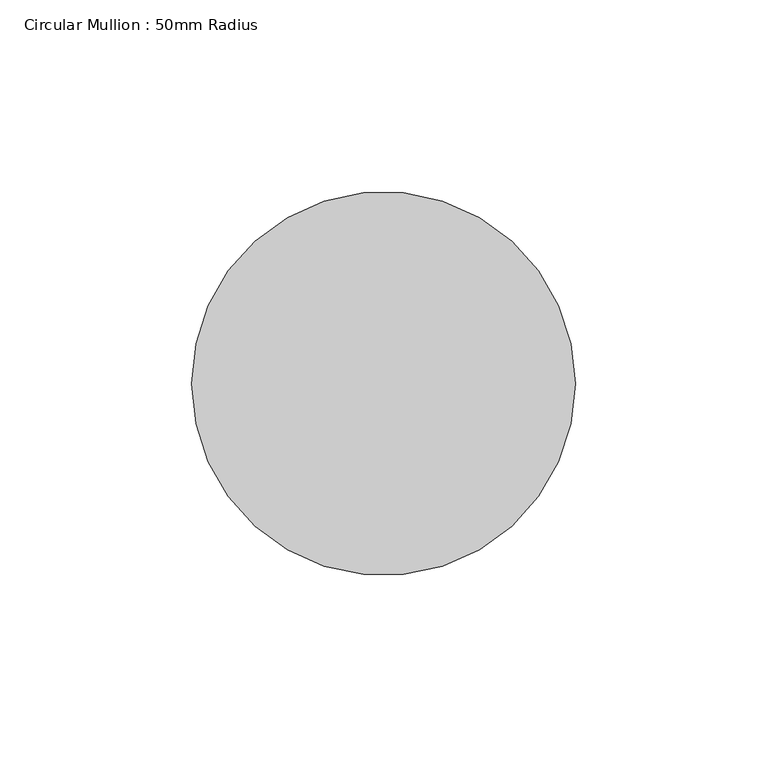
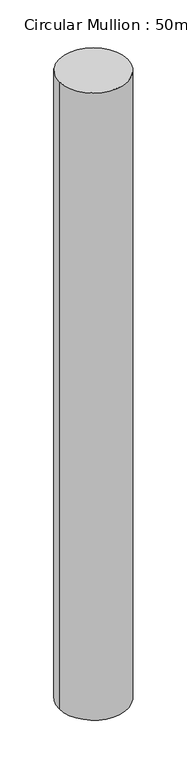
"""IFC4 building model written with IfcOpenShell, lengths in millimetres: member geometry, Circular Mullion : 50mm Radius."""

from ifc_helpers import new_model, si_unit, point, frame, origin, origin_2d, place, context, project, spatial, circle_curve, trimmed, segment, composite_curve, outline, extrude, source, transform, mapped, element, save


def circular_mullion_50mm_radius_ab17bbfe(model_context):
    return source(origin(), model_context, "Body", "SweptSolid", [
        extrude(outline(composite_curve([segment(trimmed(circle_curve(origin_2d(), 50.0), [point((50.0, 0.0))], [point((-50.0, 0.0))], False, "CARTESIAN"), True, "CONTINUOUS"), segment(trimmed(circle_curve(origin_2d(), 50.0), [point((-50.0, 0.0))], [point((50.0, 0.0))], False, "CARTESIAN"), True, "CONTINUOUS")], self_intersect=False)), frame((0.0, 0.0, -970.2752675), z_axis=(0.0, 0.0, 1.0), x_axis=(1.0, 0.0, 0.0)), (0.0, 0.0, 1.0), 970.2752675),
    ])


if __name__ == "__main__":
    model = new_model("IFC4")
    model_context = context("Model", 3, world=origin())
    ifc_project = project(units=[si_unit("LENGTHUNIT", "METRE", prefix="MILLI")], contexts=[model_context])
    site = spatial("IfcSite", under=ifc_project)
    building = spatial("IfcBuilding", under=site)
    placement = place(None, origin())
    circular_mullion_50mm_radius_shape = circular_mullion_50mm_radius_ab17bbfe(model_context)
    element("IfcMember", 1, ObjectType="Circular Mullion : 50mm Radius", at=placement, inside=building, context=model_context, shape_type="MappedRepresentation", body=[
        mapped(circular_mullion_50mm_radius_shape, transform((0.0, 0.0, 0.0), x_axis=(1.0, 0.0, 0.0), y_axis=(0.0, 1.0, 0.0), z_axis=(0.0, 0.0, 1.0))),
    ])
    save(model, "model.ifc")

# Revit data of these elements
# Type "Circular Mullion : 50mm Radius"
#   built-in parameter 1007350 = 0.164042 (stored number, unit not read)
# Element 1 (IfcMember, "Circular Mullion : 50mm Radius")
#   Materials on its faces: "Aluminium"
# Materials
#   "Aluminium": class "Metal", colour RGB 247 247 247, transparency 0, Description = "Aluminium 6061", Cost = 0
